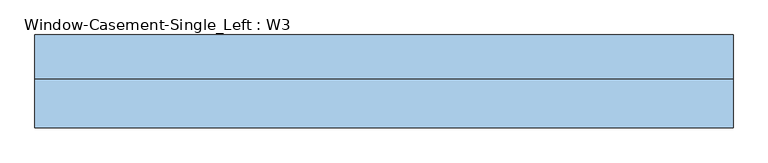
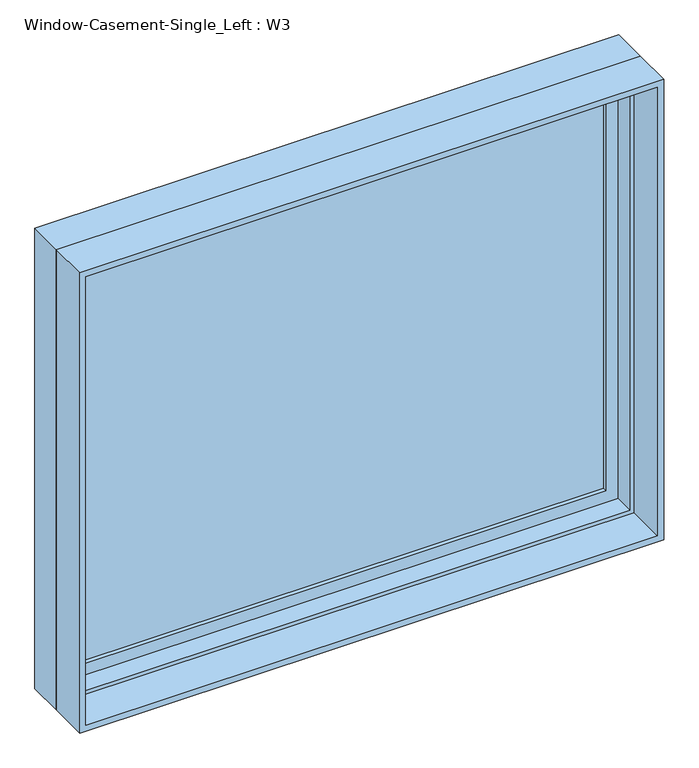
"""IFC4 building model written with IfcOpenShell, lengths in millimetres: window geometry, Window-Casement-Single_Left : W3."""

from ifc_helpers import new_model, si_unit, frame, origin, place, context, project, spatial, polyline, outline, extrude, faceted_brep, source, transform, mapped, element, save


def window_casement_single_left_w3_962045ce(model_context):
    return source(origin(), model_context, "Body", "SolidModel", [
        extrude(outline(polyline([(830.15, 110.0), (830.15, 103.65), (-830.15, 103.65), (-830.15, 110.0), (830.15, 110.0)])), frame((0.0, 0.0, 984.25), z_axis=(0.0, 0.0, 1.0), x_axis=(1.0, 0.0, 0.0)), (0.0, 0.0, 1.0), 1360.3),
        extrude(outline(polyline([(-830.15, 90.95), (-830.15, 97.3), (830.15, 97.3), (830.15, 90.95), (-830.15, 90.95)])), frame((0.0, 0.0, 984.25), z_axis=(0.0, 0.0, 1.0), x_axis=(1.0, 0.0, 0.0)), (0.0, 0.0, 1.0), 1360.3),
        extrude(outline(polyline([(2401.7, -887.3), (927.1, -887.3), (927.1, 887.3), (2401.7, 887.3), (2401.7, -887.3)]), holes=[polyline([(2344.55, 830.15), (984.25, 830.15), (984.25, -830.15), (2344.55, -830.15), (2344.55, 830.15)])]), frame((0.0, 78.25, 0.0), z_axis=(0.0, 1.0, 0.0), x_axis=(0.0, 0.0, 1.0)), (0.0, 0.0, 1.0), 44.45),
        extrude(outline(polyline([(2414.4, -900.0), (914.4, -900.0), (914.4, 900.0), (2414.4, 900.0), (2414.4, -900.0)]), holes=[polyline([(2395.35, 880.95), (933.45, 880.95), (933.45, -880.95), (2395.35, -880.95), (2395.35, 880.95)])]), frame((0.0, -110.0, 0.0), z_axis=(0.0, 1.0, 0.0), x_axis=(0.0, 0.0, 1.0)), (0.0, 0.0, 1.0), 124.75),
        faceted_brep([(868.25, 78.25, 2382.65), (868.25, 14.75, 2382.65), (-868.25, 14.75, 2382.65), (-868.25, 78.25, 2382.65), (887.3, 129.05, 2401.7), (887.3, 78.25, 2401.7), (-887.3, 78.25, 2401.7), (-887.3, 129.05, 2401.7), (900.0, 14.75, 2414.4), (900.0, 129.05, 2414.4), (-900.0, 129.05, 2414.4), (-900.0, 14.75, 2414.4), (-868.25, 14.75, 946.15), (-868.25, 78.25, 946.15), (-887.3, 78.25, 927.1), (-887.3, 129.05, 927.1), (-900.0, 129.05, 914.4), (-900.0, 14.75, 914.4), (868.25, 14.75, 946.15), (868.25, 78.25, 946.15), (887.3, 78.25, 927.1), (887.3, 129.05, 927.1), (900.0, 129.05, 914.4), (900.0, 14.75, 914.4)], [[[0, 1, 2, 3]], [[4, 5, 6, 7]], [[8, 9, 10, 11]], [[3, 2, 12, 13]], [[7, 6, 14, 15]], [[11, 10, 16, 17]], [[13, 12, 18, 19]], [[15, 14, 20, 21]], [[17, 16, 22, 23]], [[11, 17, 23, 8], [1, 18, 12, 2]], [[19, 18, 1, 0]], [[5, 20, 14, 6], [3, 13, 19, 0]], [[21, 20, 5, 4]], [[23, 22, 9, 8]], [[9, 22, 16, 10], [7, 15, 21, 4]]]),
    ])


if __name__ == "__main__":
    model = new_model("IFC4")
    model_context = context("Model", 3, world=origin())
    ifc_project = project(units=[si_unit("LENGTHUNIT", "METRE", prefix="MILLI")], contexts=[model_context])
    site = spatial("IfcSite", under=ifc_project)
    building = spatial("IfcBuilding", under=site)
    placement = place(None, origin())
    window_casement_single_left_w3_shape = window_casement_single_left_w3_962045ce(model_context)
    element("IfcWindow", 1, ObjectType="Window-Casement-Single_Left : W3", at=placement, inside=building, context=model_context, shape_type="MappedRepresentation", body=[
        mapped(window_casement_single_left_w3_shape, transform((0.0, 0.0, 0.0), x_axis=(1.0, 0.0, 0.0), y_axis=(0.0, 1.0, 0.0), z_axis=(0.0, 0.0, 1.0))),
    ])
    save(model, "model.ifc")

# Revit data of these elements
# Type "Window-Casement-Single_Left : W3"
#   Type Mark = "31"
#   Fire Rating = "0.5h"
#   Assembly Code = "B2020100"
#   Analytic Construction = "Double glazing - domestic"
#   Window Inset [instance default] = 0 cm
#   Wall Thickness [instance default] = 15.24 cm
#   Visual Light Transmittance = 0.81
#   Thermal Resistance (R) = 0.319569 (m²·K)/W
#   Solar Heat Gain Coefficient = 0.76
#   Rough Width = 181.27 cm
#   Rough Height = 151.27 cm
#   Interior Wall Closure [instance default] = 5.715 cm
#   Height = 150 cm
#   Heat Transfer Coefficient (U) = 3.12929 W/(m²·K)
#   Frame Extension [instance default] = 0.635 cm
#   Exterior Wall Closure [instance default] = 3.175 cm
#   Extension Jamb [instance default] = 5.715 cm
#   Default Sill Height = 91.44 cm
#   Width = 180 cm
#   Muntin Visibility = yes
#   Interior Trim Visibility [instance default] = yes
#   Exterior Trim Visibility [instance default] = yes
#   Extension Jamb Visibility [instance default] = yes
#   Muntin Pattern = Muntin Pattern_2x2 : Muntin Pattern_2x2
#   Interior Trim Material = Wood - Stained
#   Interior Trim = Trim-Window-Interior-Flat : Picture Frame
#   Interior Frame Material = Wood - Stained
#   Glass Panel Material = Glass
#   Exterior Trim Material = Clad - White
#   Exterior Trim = Trim-Window-Exterior-Flat : with Sill
#   Exterior Frame Material = Clad - White
#   Wall Closure = (empty or 0)
# Element 1 (IfcWindow, "Window-Casement-Single_Left : W3")
#   Wall Thickness = 22 cm
#   Extension Jamb = 12.475 cm
#   Materials on its faces: "Wood - Stained", "Glass", "Clad - White"
# Materials
#   "Wood - Stained": class "Wood", colour RGB 224 178 126, transparency 0, Cost = 0
#   "Glass": class "Glass", colour RGB 0 128 192, transparency 0.9, Description = "Soda Lime Glass", Cost = 0
#   "Clad - White": class "Wood", colour RGB 242 242 238, transparency 0, Cost = 0
